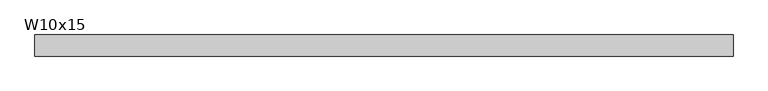
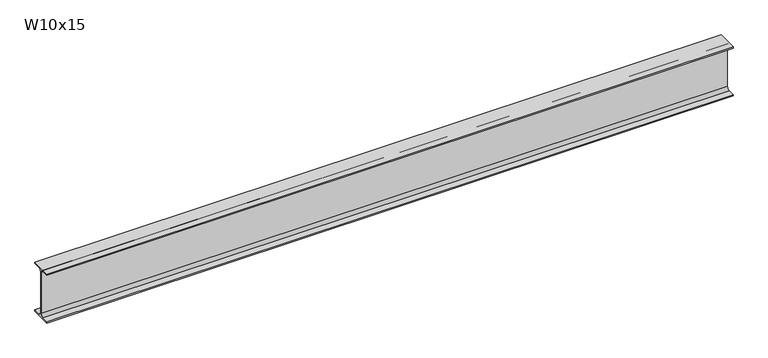
"""IFC4 building model written with IfcOpenShell, lengths in millimetres: beam geometry, RME W-Wide Flange : W10x15."""

from ifc_helpers import new_model, si_unit, point, frame, frame_2d, origin, place, context, project, spatial, polyline, circle_curve, trimmed, segment, composite_curve, outline, extrude, source, transform, mapped, element, save


def w10x15_83b6f769(model_context):
    return source(origin(), model_context, "Body", "SweptSolid", [
        extrude(outline(composite_curve([segment(polyline([(50.8, -120.142), (50.8, -127.0), (-50.8, -127.0), (-50.8, -120.142), (-16.7005, -120.142)]), True, "CONTINUOUS"), segment(trimmed(circle_curve(frame_2d((-16.7005, -106.3625)), 13.7795), [point((-16.7005, -120.142))], [point((-2.921, -106.3625))], True, "CARTESIAN"), True, "CONTINUOUS"), segment(polyline([(-2.921, -106.3625), (-2.921, 106.3625)]), True, "CONTINUOUS"), segment(trimmed(circle_curve(frame_2d((-16.7005, 106.3625)), 13.7795), [point((-2.921, 106.3625))], [point((-16.7005, 120.142))], True, "CARTESIAN"), True, "CONTINUOUS"), segment(polyline([(-16.7005, 120.142), (-50.8, 120.142), (-50.8, 127.0), (50.8, 127.0), (50.8, 120.142), (16.7005, 120.142)]), True, "CONTINUOUS"), segment(trimmed(circle_curve(frame_2d((16.7005, 106.3625)), 13.7795), [point((16.7005, 120.142))], [point((2.921, 106.3625))], True, "CARTESIAN"), True, "CONTINUOUS"), segment(polyline([(2.921, 106.3625), (2.921, -106.3625)]), True, "CONTINUOUS"), segment(trimmed(circle_curve(frame_2d((16.7005, -106.3625)), 13.7795), [point((2.921, -106.3625))], [point((16.7005, -120.142))], True, "CARTESIAN"), True, "CONTINUOUS"), segment(polyline([(16.7005, -120.142), (50.8, -120.142)]), True, "CONTINUOUS")], self_intersect=False)), frame((-1681.2922405, 0.0, 0.0), z_axis=(1.0, 0.0, 0.0), x_axis=(0.0, 1.0, 0.0)), (0.0, 0.0, 1.0), 3362.584481),
    ])


if __name__ == "__main__":
    model = new_model("IFC4")
    model_context = context("Model", 3, world=origin())
    ifc_project = project(units=[si_unit("LENGTHUNIT", "METRE", prefix="MILLI")], contexts=[model_context])
    site = spatial("IfcSite", under=ifc_project)
    building = spatial("IfcBuilding", under=site)
    placement = place(None, origin())
    w10x15_shape = w10x15_83b6f769(model_context)
    element("IfcBeam", 1, ObjectType="RME W-Wide Flange : W10x15", at=placement, inside=building, context=model_context, shape_type="MappedRepresentation", body=[
        mapped(w10x15_shape, transform((0.0, 0.0, 0.0), x_axis=(1.0, 0.0, 0.0), y_axis=(0.0, 1.0, 0.0), z_axis=(0.0, 0.0, 1.0))),
    ])
    save(model, "model.ifc")

# Revit data of these elements
# Type "RME W-Wide Flange : W10x15"
#   WELD P [instance default] = ""
#   WELD LE [instance default] = ""
#   WELD D [instance default] = ""
#   TOP SECTION SIZE [instance default] = ""
#   TOP SECTION LENGTH [instance default] = ""
#   REMARKS [instance default] = ""
#   REINF TYPE [instance default] = ""
#   Nominal Size = "W24"
#   End Bearing Capacity [instance default] = ""
#   BOT SECTION SIZE [instance default] = ""
#   BOT SECTION LENGTH [instance default] = ""
#   Assembly Code = "B10"
#   W = 15
#   Start Extension Calculation [instance default] = 10' - 0"
#   Start Extension [instance default] = -0' - 0 1/2"
#   End Extension Calculation [instance default] = 10' - 0"
#   End Extension [instance default] = -0' - 0 1/2"
#   Length [instance default] = 5' - 0"
#   bf = 0' - 4"
#   d = 0' - 10"
#   k = 0' - 0 13/16"
#   k2 = 0' - 0.5425"
#   tf = 0' - 0.27"
#   tw = 0' - 0.23"
#   A = 0.030625 SF
#   Structural Material [instance default] = Metal - Steel - ASTM A992
# Element 1 (IfcBeam, "RME W-Wide Flange : W10x15")
#   Length = 11' - 0.38522"
#   Materials on its faces: "Metal - Steel - ASTM A992"
# Materials
#   "Metal - Steel - ASTM A992": class "Metal", colour RGB 255 128 0, transparency 0
